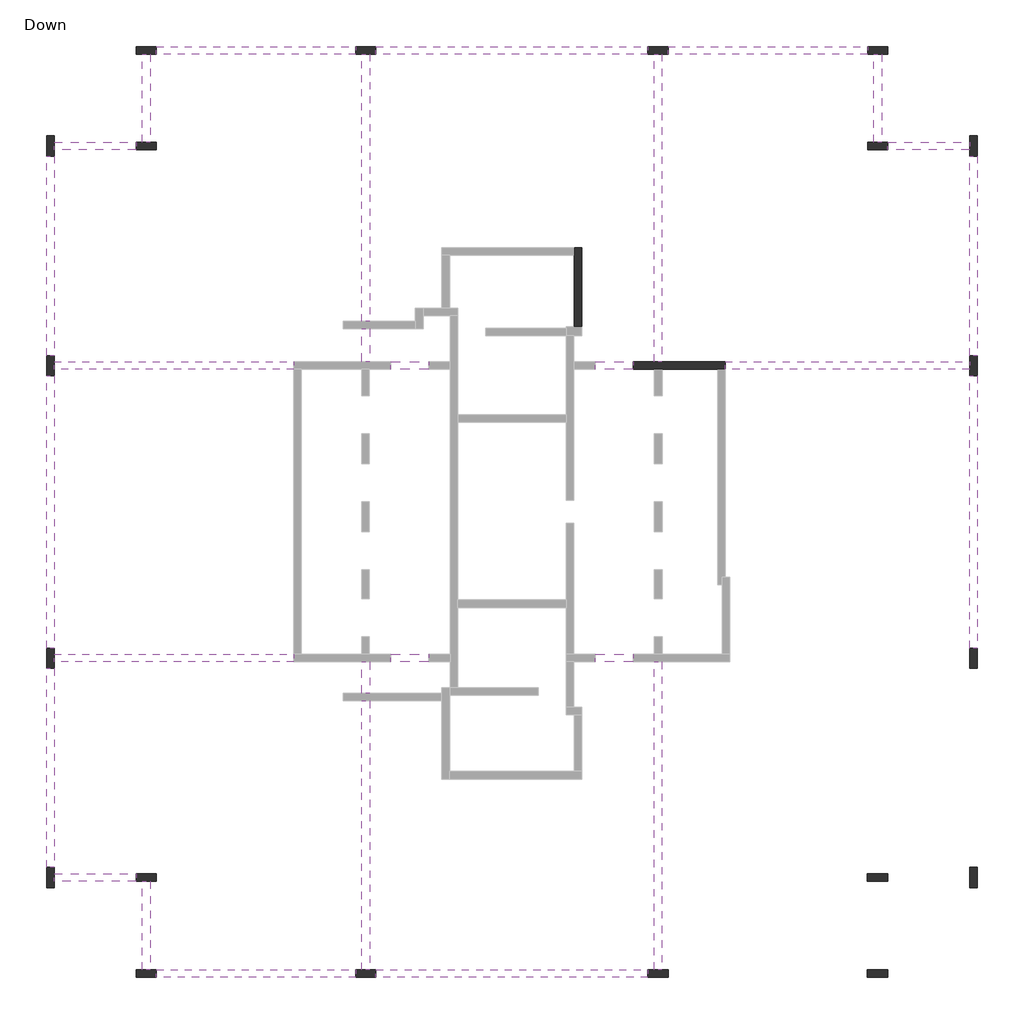
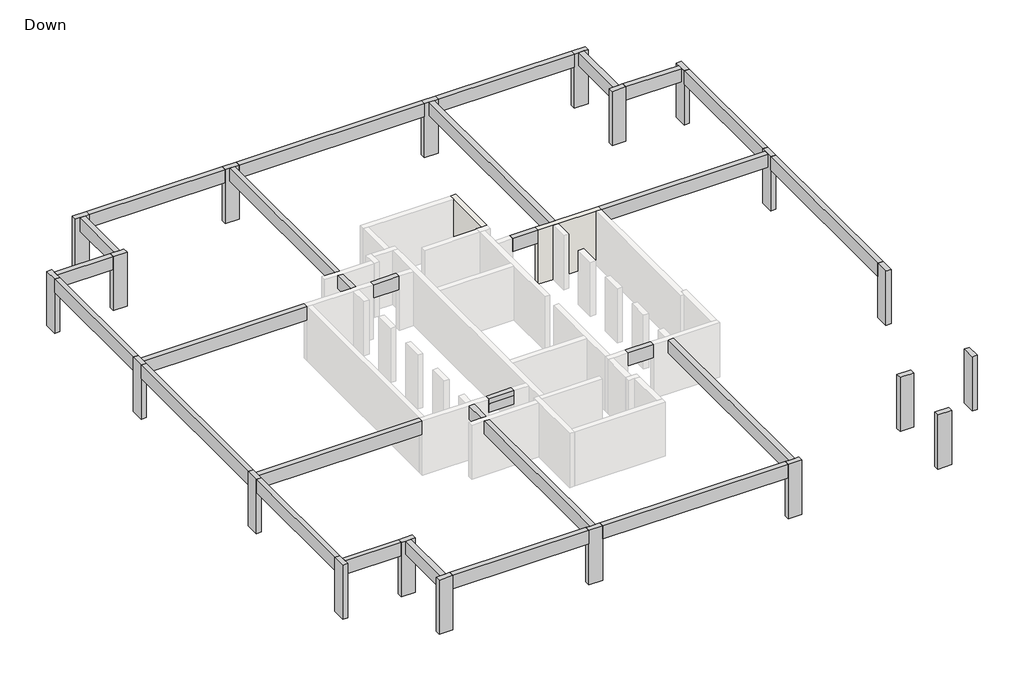
# One storey, part 2 of 2: 29 beams, 20 columns, 2 walls.
"""IFC4 building model written with IfcOpenShell, lengths in millimetres."""

from ifc_helpers import new_model, si_unit, frame, origin, place, context, project, spatial, polyline, outline, extrude, faceted_brep, element, save

model = new_model("IFC4")

# Units and contexts
model_context = context("Model", 3, world=origin())
ifc_project = project(units=[si_unit("LENGTHUNIT", "METRE", prefix="MILLI")], contexts=[model_context])

# Site, building, storey
site = spatial("IfcSite", under=ifc_project)
building = spatial("IfcBuilding", under=site)
storey = spatial("IfcBuildingStorey", under=building, Name="Down", Elevation=0.0)

# Beams
placement = place(None, origin())
element("IfcBeam", 1, ObjectType="Concrete Rectengular Beam : 30/80", at=placement, inside=storey, context=model_context, shape_type="SweptSolid", body=[
    extrude(outline(polyline([(-18816.7874799, -2513.9587131), (-18516.7874799, -2513.9587131), (-18516.7874799, -10341.2814935), (-18816.7874799, -10341.2814935), (-18816.7874799, -2513.9587131)])), frame((0.0, 0.0, 2500.0), z_axis=(0.0, 0.0, 1.0), x_axis=(1.0, 0.0, 0.0)), (0.0, 0.0, 1.0), 800.0),
])
element("IfcBeam", 2, ObjectType="Concrete Rectengular Beam : 30/80", at=placement, inside=storey, context=model_context, shape_type="Brep", body=[
    faceted_brep([(-18516.7874799, -10591.2814935, 3300.0), (-18516.7874799, -10891.2814935, 3300.0), (-15296.5493178, -10891.2814935, 3300.0), (-15296.5493178, -10591.2814935, 3300.0), (-18516.7874799, -10891.2814935, 3000.0), (-18516.7874799, -10891.2814935, 2500.0), (-15296.5493178, -10891.2814935, 2500.0), (-18516.7874799, -10591.2814935, 2500.0), (-15296.5493178, -10591.2814935, 2500.0), (-15296.5493178, -10591.2814935, 3000.0), (-18516.7874799, -10591.2814935, 3000.0)], [[[0, 1, 2, 3]], [[1, 4, 5, 6, 2]], [[5, 7, 8, 6]], [[0, 3, 9, 8, 7, 10]], [[5, 4, 1, 0, 10, 7]], [[3, 2, 6, 8, 9]]]),
])
element("IfcBeam", 3, ObjectType="Concrete Rectengular Beam : 30/80", at=placement, inside=storey, context=model_context, shape_type="Brep", body=[
    faceted_brep([(-14746.5493178, -10891.2814935, 3300.0), (-15046.5493178, -10891.2814935, 3300.0), (-15046.5493178, -14364.3468097, 3300.0), (-14746.5493178, -14364.3468097, 3300.0), (-14746.5493178, -14364.3468097, 3000.0), (-14746.5493178, -14364.3468097, 2500.0), (-14746.5493178, -10891.2814935, 2500.0), (-14746.5493178, -10891.2814935, 3000.0), (-15046.5493178, -10891.2814935, 2500.0), (-15046.5493178, -14364.3468097, 2500.0), (-15046.5493178, -10891.2814935, 3000.0), (-15046.5493178, -14364.3468097, 3000.0)], [[[0, 1, 2, 3]], [[0, 3, 4, 5, 6, 7]], [[8, 6, 5, 9]], [[1, 10, 8, 9, 11, 2]], [[8, 10, 1, 0, 7, 6]], [[3, 2, 11, 9, 5, 4]]]),
])
element("IfcBeam", 4, ObjectType="Concrete Rectengular Beam : 30/80", at=placement, inside=storey, context=model_context, shape_type="SweptSolid", body=[
    extrude(outline(polyline([(-14496.5493178, -14664.3468097), (-14496.5493178, -14364.3468097), (-6665.2243211, -14364.3468097), (-6665.2243211, -14664.3468097), (-14496.5493178, -14664.3468097)])), frame((0.0, 0.0, 2500.0), z_axis=(0.0, 0.0, 1.0), x_axis=(1.0, 0.0, 0.0)), (0.0, 0.0, 1.0), 800.0),
])
element("IfcBeam", 5, ObjectType="Concrete Rectengular Beam : 30/80", at=placement, inside=storey, context=model_context, shape_type="Brep", body=[
    faceted_brep([(-18516.7874799, -1956.2642878, 3300.0), (-18516.7874799, -2256.2642878, 3300.0), (-9097.9299438, -2256.2642878, 3300.0), (-9097.9299438, -1956.2642878, 3300.0), (-18516.7874799, -1956.2642878, 2500.0), (-18516.7874799, -1956.2642878, 3000.0), (-9097.9299438, -1956.2642878, 3000.0), (-9097.9299438, -1956.2642878, 2500.0), (-18516.7874799, -2256.2642878, 2500.0), (-9097.9299438, -2256.2642878, 2500.0), (-18516.7874799, -2256.2642878, 3000.0)], [[[0, 1, 2, 3]], [[4, 5, 0, 3, 6, 7]], [[8, 4, 7, 9]], [[1, 10, 8, 9, 2]], [[8, 10, 1, 0, 5, 4]], [[3, 2, 9, 7, 6]]]),
])
element("IfcBeam", 6, ObjectType="Concrete Rectengular Beam : 30/80", at=placement, inside=storey, context=model_context, shape_type="SweptSolid", body=[
    extrude(outline(polyline([(-18516.7874799, -1713.9587131), (-18816.7874799, -1713.9587131), (-18816.7874799, 8986.0412869), (-18516.7874799, 8986.0412869), (-18516.7874799, -1713.9587131)])), frame((0.0, 0.0, 2500.0), z_axis=(0.0, 0.0, 1.0), x_axis=(1.0, 0.0, 0.0)), (0.0, 0.0, 1.0), 800.0),
])
element("IfcBeam", 7, ObjectType="Concrete Rectengular Beam : 30/80", at=placement, inside=storey, context=model_context, shape_type="Brep", body=[
    faceted_brep([(-18516.7874799, 9551.0309634, 3300.0), (-18516.7874799, 9251.0309634, 3300.0), (-9097.9299438, 9251.0309634, 3300.0), (-9097.9299438, 9551.0309634, 3300.0), (-18516.7874799, 9251.0309634, 3000.0), (-18516.7874799, 9251.0309634, 2500.0), (-9097.9299438, 9251.0309634, 2500.0), (-9097.9299438, 9251.0309634, 3000.0), (-18516.7874799, 9551.0309634, 2500.0), (-9097.9299438, 9551.0309634, 2500.0), (-18516.7874799, 9551.0309634, 3000.0)], [[[0, 1, 2, 3]], [[1, 4, 5, 6, 7, 2]], [[5, 8, 9, 6]], [[8, 10, 0, 3, 9]], [[5, 4, 1, 0, 10, 8]], [[3, 2, 7, 6, 9]]]),
])
element("IfcBeam", 8, ObjectType="Concrete Rectengular Beam : 30/80", at=placement, inside=storey, context=model_context, shape_type="SweptSolid", body=[
    extrude(outline(polyline([(-18516.7874799, 9786.0412869), (-18816.7874799, 9786.0412869), (-18816.7874799, 17624.5114627), (-18516.7874799, 17624.5114627), (-18516.7874799, 9786.0412869)])), frame((0.0, 0.0, 2500.0), z_axis=(0.0, 0.0, 1.0), x_axis=(1.0, 0.0, 0.0)), (0.0, 0.0, 1.0), 800.0),
])
element("IfcBeam", 9, ObjectType="Concrete Rectengular Beam : 30/80", at=placement, inside=storey, context=model_context, shape_type="Brep", body=[
    faceted_brep([(-15046.5493178, 18174.5114627, 3300.0), (-14746.5493178, 18174.5114627, 3300.0), (-14746.5493178, 21634.8017643, 3300.0), (-15046.5493178, 21634.8017643, 3300.0), (-14746.5493178, 18174.5114627, 3000.0), (-14746.5493178, 18174.5114627, 2500.0), (-14746.5493178, 21634.8017643, 2500.0), (-14746.5493178, 21634.8017643, 3000.0), (-15046.5493178, 18174.5114627, 2500.0), (-15046.5493178, 21634.8017643, 2500.0), (-15046.5493178, 18174.5114627, 3000.0), (-15046.5493178, 21634.8017643, 3000.0)], [[[0, 1, 2, 3]], [[2, 1, 4, 5, 6, 7]], [[5, 8, 9, 6]], [[8, 10, 0, 3, 11, 9]], [[1, 0, 10, 8, 5, 4]], [[3, 2, 7, 6, 9, 11]]]),
])
element("IfcBeam", 10, ObjectType="Concrete Rectengular Beam : 30/80", at=placement, inside=storey, context=model_context, shape_type="Brep", body=[
    faceted_brep([(-6115.2243211, 21634.8017643, 3300.0), (-6415.2243211, 21634.8017643, 3300.0), (-6415.2243211, 11137.9545698, 3300.0), (-6115.2243211, 11137.9545698, 3300.0), (-6415.2243211, 21634.8017643, 3000.0), (-6415.2243211, 21634.8017643, 2500.0), (-6415.2243211, 11137.9545698, 2500.0), (-6415.2243211, 11137.9545698, 3000.0), (-6115.2243211, 21634.8017643, 2500.0), (-6115.2243211, 11137.9545698, 2500.0), (-6115.2243211, 21634.8017643, 3000.0), (-6115.2243211, 11137.9545698, 3000.0)], [[[0, 1, 2, 3]], [[1, 4, 5, 6, 7, 2]], [[5, 8, 9, 6]], [[8, 10, 0, 3, 11, 9]], [[1, 0, 10, 8, 5, 4]], [[3, 2, 7, 6, 9, 11]]]),
])
element("IfcBeam", 11, ObjectType="Concrete Rectengular Beam : 30/80", at=placement, inside=storey, context=model_context, shape_type="SweptSolid", body=[
    extrude(outline(polyline([(-5865.2243211, 21634.8017643), (-5865.2243211, 21934.8017643), (4823.25294, 21934.8017643), (4823.25294, 21634.8017643), (-5865.2243211, 21634.8017643)])), frame((0.0, 0.0, 2500.0), z_axis=(0.0, 0.0, 1.0), x_axis=(1.0, 0.0, 0.0)), (0.0, 0.0, 1.0), 800.0),
])
element("IfcBeam", 12, ObjectType="Concrete Rectengular Beam : 30/80", at=placement, inside=storey, context=model_context, shape_type="Brep", body=[
    faceted_brep([(14014.5779368, 21634.8017643, 3300.0), (13714.5779368, 21634.8017643, 3300.0), (13714.5779368, 18174.5114627, 3300.0), (14014.5779368, 18174.5114627, 3300.0), (13714.5779368, 21634.8017643, 3000.0), (13714.5779368, 21634.8017643, 2500.0), (13714.5779368, 18174.5114627, 2500.0), (13714.5779368, 18174.5114627, 3000.0), (14014.5779368, 21634.8017643, 2500.0), (14014.5779368, 18174.5114627, 2500.0), (14014.5779368, 21634.8017643, 3000.0), (14014.5779368, 18174.5114627, 3000.0)], [[[0, 1, 2, 3]], [[2, 1, 4, 5, 6, 7]], [[5, 8, 9, 6]], [[8, 10, 0, 3, 11, 9]], [[1, 0, 10, 8, 5, 4]], [[3, 2, 7, 6, 9, 11]]]),
])
element("IfcBeam", 13, ObjectType="Concrete Rectengular Beam : 30/80", at=placement, inside=storey, context=model_context, shape_type="SweptSolid", body=[
    extrude(outline(polyline([(17474.8160989, 17624.5114627), (17774.8160989, 17624.5114627), (17774.8160989, 9786.0412869), (17474.8160989, 9786.0412869), (17474.8160989, 17624.5114627)])), frame((0.0, 0.0, 2500.0), z_axis=(0.0, 0.0, 1.0), x_axis=(1.0, 0.0, 0.0)), (0.0, 0.0, 1.0), 800.0),
])
element("IfcBeam", 14, ObjectType="Concrete Rectengular Beam : 30/80", at=placement, inside=storey, context=model_context, shape_type="SweptSolid", body=[
    extrude(outline(polyline([(17774.8160989, -1713.9587131), (17474.8160989, -1713.9587131), (17474.8160989, 8986.0412869), (17774.8160989, 8986.0412869), (17774.8160989, -1713.9587131)])), frame((0.0, 0.0, 2500.0), z_axis=(0.0, 0.0, 1.0), x_axis=(1.0, 0.0, 0.0)), (0.0, 0.0, 1.0), 800.0),
])
element("IfcBeam", 15, ObjectType="Concrete Rectengular Beam : 30/80", at=placement, inside=storey, context=model_context, shape_type="Brep", body=[
    faceted_brep([(14264.5779368, 18174.5114627, 3300.0), (14264.5779368, 17874.5114627, 3300.0), (17474.8160989, 17874.5114627, 3300.0), (17474.8160989, 18174.5114627, 3300.0), (14264.5779368, 18174.5114627, 2500.0), (17474.8160989, 18174.5114627, 3000.0), (17474.8160989, 18174.5114627, 2500.0), (14264.5779368, 17874.5114627, 2500.0), (17474.8160989, 17874.5114627, 2500.0), (14264.5779368, 17874.5114627, 3000.0), (17474.8160989, 17874.5114627, 3000.0)], [[[0, 1, 2, 3]], [[4, 0, 3, 5, 6]], [[7, 4, 6, 8]], [[2, 1, 9, 7, 8, 10]], [[1, 0, 4, 7, 9]], [[6, 5, 3, 2, 10, 8]]]),
])
element("IfcBeam", 16, ObjectType="Concrete Rectengular Beam : 30/80", at=placement, inside=storey, context=model_context, shape_type="SweptSolid", body=[
    extrude(outline(polyline([(5623.25294, 21634.8017643), (5623.25294, 21934.8017643), (13464.5779368, 21934.8017643), (13464.5779368, 21634.8017643), (5623.25294, 21634.8017643)])), frame((0.0, 0.0, 2500.0), z_axis=(0.0, 0.0, 1.0), x_axis=(1.0, 0.0, 0.0)), (0.0, 0.0, 1.0), 800.0),
])
element("IfcBeam", 17, ObjectType="Concrete Rectengular Beam : 30/80", at=placement, inside=storey, context=model_context, shape_type="SweptSolid", body=[
    extrude(outline(polyline([(-5865.2243211, -14664.3468097), (-5865.2243211, -14364.3468097), (4823.25294, -14364.3468097), (4823.25294, -14664.3468097), (-5865.2243211, -14664.3468097)])), frame((0.0, 0.0, 2500.0), z_axis=(0.0, 0.0, 1.0), x_axis=(1.0, 0.0, 0.0)), (0.0, 0.0, 1.0), 800.0),
])
element("IfcBeam", 18, ObjectType="Concrete Rectengular Beam : 30/80", at=placement, inside=storey, context=model_context, shape_type="Brep", body=[
    faceted_brep([(-6415.2243211, -14364.3468097, 3300.0), (-6115.2243211, -14364.3468097, 3300.0), (-6115.2243211, -3792.8093669, 3300.0), (-6415.2243211, -3792.8093669, 3300.0), (-6115.2243211, -14364.3468097, 3000.0), (-6115.2243211, -14364.3468097, 2500.0), (-6115.2243211, -3792.8093669, 2500.0), (-6115.2243211, -3792.8093669, 3000.0), (-6415.2243211, -14364.3468097, 2500.0), (-6415.2243211, -3792.8093669, 2500.0), (-6415.2243211, -14364.3468097, 3000.0), (-6415.2243211, -3792.8093669, 3000.0)], [[[0, 1, 2, 3]], [[1, 4, 5, 6, 7, 2]], [[5, 8, 9, 6]], [[8, 10, 0, 3, 11, 9]], [[0, 10, 8, 5, 4, 1]], [[3, 2, 7, 6, 9, 11]]]),
])
element("IfcBeam", 19, ObjectType="Concrete Rectengular Beam : 30/80", at=placement, inside=storey, context=model_context, shape_type="Brep", body=[
    faceted_brep([(-6115.2243211, -2256.2642878, 3300.0), (-6415.2243211, -2256.2642878, 3300.0), (-6415.2243211, -3492.8093669, 3300.0), (-6115.2243211, -3492.8093669, 3300.0), (-6115.2243211, -2256.2642878, 2500.0), (-6115.2243211, -2256.2642878, 3000.0), (-6115.2243211, -3492.8093669, 3000.0), (-6115.2243211, -3492.8093669, 2500.0), (-6415.2243211, -2256.2642878, 2500.0), (-6415.2243211, -3492.8093669, 2500.0), (-6415.2243211, -2256.2642878, 3000.0), (-6415.2243211, -3492.8093669, 3000.0)], [[[0, 1, 2, 3]], [[4, 5, 0, 3, 6, 7]], [[8, 4, 7, 9]], [[1, 10, 8, 9, 11, 2]], [[1, 0, 5, 4, 8, 10]], [[3, 2, 11, 9, 7, 6]]]),
])
element("IfcBeam", 20, ObjectType="Concrete Rectengular Beam : 30/80", at=placement, inside=storey, context=model_context, shape_type="Brep", body=[
    faceted_brep([(5073.25294, -14364.3468097, 3300.0), (5373.25294, -14364.3468097, 3300.0), (5373.25294, -2256.2642878, 3300.0), (5073.25294, -2256.2642878, 3300.0), (5073.25294, -14364.3468097, 2500.0), (5073.25294, -14364.3468097, 3000.0), (5073.25294, -2256.2642878, 3000.0), (5073.25294, -2256.2642878, 2500.0), (5373.25294, -14364.3468097, 2500.0), (5373.25294, -2256.2642878, 2500.0), (5373.25294, -14364.3468097, 3000.0), (5373.25294, -2256.2642878, 3000.0)], [[[0, 1, 2, 3]], [[4, 5, 0, 3, 6, 7]], [[8, 4, 7, 9]], [[1, 10, 8, 9, 11, 2]], [[8, 10, 1, 0, 5, 4]], [[3, 2, 11, 9, 7, 6]]]),
])
element("IfcBeam", 21, ObjectType="Concrete Rectengular Beam : 30/80", at=placement, inside=storey, context=model_context, shape_type="Brep", body=[
    faceted_brep([(-18516.7874799, 18174.5114627, 3300.0), (-18516.7874799, 17874.5114627, 3300.0), (-15296.5493178, 17874.5114627, 3300.0), (-15296.5493178, 18174.5114627, 3300.0), (-18516.7874799, 17874.5114627, 3000.0), (-18516.7874799, 17874.5114627, 2500.0), (-15296.5493178, 17874.5114627, 2500.0), (-15296.5493178, 17874.5114627, 3000.0), (-18516.7874799, 18174.5114627, 2500.0), (-15296.5493178, 18174.5114627, 2500.0), (-18516.7874799, 18174.5114627, 3000.0)], [[[0, 1, 2, 3]], [[2, 1, 4, 5, 6, 7]], [[5, 8, 9, 6]], [[8, 10, 0, 3, 9]], [[0, 10, 8, 5, 4, 1]], [[3, 2, 7, 6, 9]]]),
])
element("IfcBeam", 22, ObjectType="Concrete Rectengular Beam : 30/80", at=placement, inside=storey, context=model_context, shape_type="SweptSolid", body=[
    extrude(outline(polyline([(-14496.5493178, 21634.8017643), (-14496.5493178, 21934.8017643), (-6665.2243211, 21934.8017643), (-6665.2243211, 21634.8017643), (-14496.5493178, 21634.8017643)])), frame((0.0, 0.0, 2500.0), z_axis=(0.0, 0.0, 1.0), x_axis=(1.0, 0.0, 0.0)), (0.0, 0.0, 1.0), 800.0),
])
element("IfcBeam", 23, ObjectType="Concrete Rectengular Beam : 30/80", at=placement, inside=storey, context=model_context, shape_type="Brep", body=[
    faceted_brep([(5373.25294, 21634.8017643, 3300.0), (5073.25294, 21634.8017643, 3300.0), (5073.25294, 9551.0309634, 3300.0), (5373.25294, 9551.0309634, 3300.0), (5073.25294, 21634.8017643, 3000.0), (5073.25294, 21634.8017643, 2500.0), (5073.25294, 9551.0309634, 2500.0), (5073.25294, 9551.0309634, 3000.0), (5373.25294, 21634.8017643, 2500.0), (5373.25294, 9551.0309634, 2500.0), (5373.25294, 21634.8017643, 3000.0), (5373.25294, 9551.0309634, 3000.0)], [[[0, 1, 2, 3]], [[1, 4, 5, 6, 7, 2]], [[5, 8, 9, 6]], [[8, 10, 0, 3, 11, 9]], [[5, 4, 1, 0, 10, 8]], [[3, 2, 7, 6, 9, 11]]]),
])
element("IfcBeam", 24, ObjectType="Concrete Rectengular Beam : 30/80", at=placement, inside=storey, context=model_context, shape_type="Brep", body=[
    faceted_brep([(17474.8160989, 9251.0309634, 3300.0), (17474.8160989, 9551.0309634, 3300.0), (7862.8408752, 9551.0309634, 3300.0), (7862.8408752, 9251.0309634, 3300.0), (17474.8160989, 9551.0309634, 3000.0), (17474.8160989, 9551.0309634, 2500.0), (7862.8408752, 9551.0309634, 2500.0), (17474.8160989, 9251.0309634, 2500.0), (7862.8408752, 9251.0309634, 2500.0), (17474.8160989, 9251.0309634, 3000.0), (7862.8408752, 9251.0309634, 3000.0)], [[[0, 1, 2, 3]], [[1, 4, 5, 6, 2]], [[5, 7, 8, 6]], [[7, 9, 0, 3, 10, 8]], [[5, 4, 1, 0, 9, 7]], [[3, 2, 6, 8, 10]]]),
])
element("IfcBeam", 25, ObjectType="Concrete Rectengular Beam : 30/80", at=placement, inside=storey, context=model_context, shape_type="SweptSolid", body=[
    extrude(outline(polyline([(2756.2889137, 9251.0309634), (2756.2889137, 9551.0309634), (4242.4554657, 9551.0309634), (4242.4554657, 9251.0309634), (2756.2889137, 9251.0309634)])), frame((0.0, 0.0, 2500.0), z_axis=(0.0, 0.0, 1.0), x_axis=(1.0, 0.0, 0.0)), (0.0, 0.0, 1.0), 800.0),
])
element("IfcBeam", 26, ObjectType="Concrete Rectengular Beam : 30/80", at=placement, inside=storey, context=model_context, shape_type="SweptSolid", body=[
    extrude(outline(polyline([(2756.2889137, -2256.2642878), (2756.2889137, -1956.2642878), (4242.4554657, -1956.2642878), (4242.4554657, -2256.2642878), (2756.2889137, -2256.2642878)])), frame((0.0, 0.0, 2500.0), z_axis=(0.0, 0.0, 1.0), x_axis=(1.0, 0.0, 0.0)), (0.0, 0.0, 1.0), 800.0),
])
element("IfcBeam", 27, ObjectType="Concrete Rectengular Beam : 30/80", at=placement, inside=storey, context=model_context, shape_type="SweptSolid", body=[
    extrude(outline(polyline([(-1956.2642878, 3300.0), (-1956.2642878, 2500.0), (-2256.2642878, 2500.0), (-2256.2642878, 3000.0), (-2251.2642878, 3000.0), (-2251.2642878, 3300.0), (-1956.2642878, 3300.0)])), frame((-5277.5582989, 0.0, 0.0), z_axis=(1.0, 0.0, 0.0), x_axis=(0.0, 1.0, 0.0)), (0.0, 0.0, 1.0), 1486.166552),
])
element("IfcBeam", 28, ObjectType="Concrete Rectengular Beam : 30/80", at=placement, inside=storey, context=model_context, shape_type="SweptSolid", body=[
    extrude(outline(polyline([(-3791.391747, 9551.0309634), (-3791.391747, 9251.0309634), (-5277.5582989, 9251.0309634), (-5277.5582989, 9551.0309634), (-3791.391747, 9551.0309634)])), frame((0.0, 0.0, 2500.0), z_axis=(0.0, 0.0, 1.0), x_axis=(1.0, 0.0, 0.0)), (0.0, 0.0, 1.0), 800.0),
])
element("IfcBeam", 29, ObjectType="Concrete Rectengular Beam : 30/80", at=placement, inside=storey, context=model_context, shape_type="Brep", body=[
    faceted_brep([(-6415.2243211, 9551.0309634, 3300.0), (-6115.2243211, 9551.0309634, 3300.0), (-6115.2243211, 10837.9545698, 3300.0), (-6415.2243211, 10837.9545698, 3300.0), (-6115.2243211, 9551.0309634, 3000.0), (-6115.2243211, 9551.0309634, 2500.0), (-6115.2243211, 10837.9545698, 2500.0), (-6115.2243211, 10837.9545698, 3000.0), (-6415.2243211, 9551.0309634, 2500.0), (-6415.2243211, 10837.9545698, 2500.0), (-6415.2243211, 9551.0309634, 3000.0), (-6415.2243211, 10837.9545698, 3000.0)], [[[0, 1, 2, 3]], [[1, 4, 5, 6, 7, 2]], [[5, 8, 9, 6]], [[8, 10, 0, 3, 11, 9]], [[1, 0, 10, 8, 5, 4]], [[3, 2, 7, 6, 9, 11]]]),
])

# Columns
element("IfcColumn", 30, ObjectType="Concrete Rectengular Column : 30/80", at=placement, inside=storey, context=model_context, shape_type="Brep", body=[
    faceted_brep([(-18516.7874799, -1713.9587131, 0.0), (-18516.7874799, -2513.9587131, 0.0), (-18816.7874799, -2513.9587131, 0.0), (-18816.7874799, -1713.9587131, 0.0), (-18516.7874799, -1713.9587131, 3300.0), (-18516.7874799, -1956.2642878, 3300.0), (-18516.7874799, -2256.2642878, 3300.0), (-18516.7874799, -2513.9587131, 3300.0), (-18816.7874799, -2513.9587131, 3300.0), (-18816.7874799, -1713.9587131, 3300.0)], [[[0, 1, 2, 3]], [[4, 5, 6, 7, 1, 0]], [[7, 8, 2, 1]], [[8, 9, 3, 2]], [[9, 4, 0, 3]], [[4, 9, 8, 7, 6, 5]]]),
])
element("IfcColumn", 31, ObjectType="Concrete Rectengular Column : 30/80", at=placement, inside=storey, context=model_context, shape_type="Brep", body=[
    faceted_brep([(-18516.7874799, -10341.2814935, 0.0), (-18516.7874799, -11141.2814935, 0.0), (-18816.7874799, -11141.2814935, 0.0), (-18816.7874799, -10341.2814935, 0.0), (-18516.7874799, -10341.2814935, 3300.0), (-18516.7874799, -10591.2814935, 3300.0), (-18516.7874799, -10891.2814935, 3300.0), (-18516.7874799, -11141.2814935, 3300.0), (-18516.7874799, -11141.2814935, 3000.0), (-18816.7874799, -11141.2814935, 3300.0), (-18816.7874799, -11141.2814935, 3000.0), (-18816.7874799, -10341.2814935, 3300.0)], [[[0, 1, 2, 3]], [[4, 5, 6, 7, 8, 1, 0]], [[7, 9, 10, 2, 1, 8]], [[9, 11, 3, 2, 10]], [[11, 4, 0, 3]], [[4, 11, 9, 7, 6, 5]]]),
])
element("IfcColumn", 32, ObjectType="Concrete Rectengular Column : 30/80", at=placement, inside=storey, context=model_context, shape_type="Brep", body=[
    faceted_brep([(-15296.5493178, -10591.2814935, 0.0), (-14496.5493178, -10591.2814935, 0.0), (-14496.5493178, -10891.2814935, 0.0), (-15296.5493178, -10891.2814935, 0.0), (-15296.5493178, -10591.2814935, 3300.0), (-14496.5493178, -10591.2814935, 3300.0), (-14496.5493178, -10591.2814935, 3000.0), (-14496.5493178, -10891.2814935, 3300.0), (-14496.5493178, -10891.2814935, 3000.0), (-14746.5493178, -10891.2814935, 3300.0), (-15046.5493178, -10891.2814935, 3300.0), (-15296.5493178, -10891.2814935, 3300.0)], [[[0, 1, 2, 3]], [[4, 5, 6, 1, 0]], [[5, 7, 8, 2, 1, 6]], [[7, 9, 10, 11, 3, 2, 8]], [[11, 4, 0, 3]], [[4, 11, 10, 9, 7, 5]]]),
])
element("IfcColumn", 33, ObjectType="Concrete Rectengular Column : 30/80", at=placement, inside=storey, context=model_context, shape_type="Brep", body=[
    faceted_brep([(-15296.5493178, -14364.3468097, 0.0), (-14496.5493178, -14364.3468097, 0.0), (-14496.5493178, -14664.3468097, 0.0), (-15296.5493178, -14664.3468097, 0.0), (-15296.5493178, -14364.3468097, 3300.0), (-15046.5493178, -14364.3468097, 3300.0), (-14746.5493178, -14364.3468097, 3300.0), (-14496.5493178, -14364.3468097, 3300.0), (-15296.5493178, -14364.3468097, 3000.0), (-14496.5493178, -14664.3468097, 3300.0), (-15296.5493178, -14664.3468097, 3300.0), (-15296.5493178, -14664.3468097, 3000.0)], [[[0, 1, 2, 3]], [[4, 5, 6, 7, 1, 0, 8]], [[7, 9, 2, 1]], [[9, 10, 11, 3, 2]], [[10, 4, 8, 0, 3, 11]], [[4, 10, 9, 7, 6, 5]]]),
])
element("IfcColumn", 34, ObjectType="Concrete Rectengular Column : 30/80", at=placement, inside=storey, context=model_context, shape_type="Brep", body=[
    faceted_brep([(-6665.2243211, -14364.3468097, 0.0), (-5865.2243211, -14364.3468097, 0.0), (-5865.2243211, -14664.3468097, 0.0), (-6665.2243211, -14664.3468097, 0.0), (-6665.2243211, -14364.3468097, 3300.0), (-6415.2243211, -14364.3468097, 3300.0), (-6115.2243211, -14364.3468097, 3300.0), (-5865.2243211, -14364.3468097, 3300.0), (-5865.2243211, -14664.3468097, 3300.0), (-6665.2243211, -14664.3468097, 3300.0)], [[[0, 1, 2, 3]], [[4, 5, 6, 7, 1, 0]], [[7, 8, 2, 1]], [[8, 9, 3, 2]], [[9, 4, 0, 3]], [[4, 9, 8, 7, 6, 5]]]),
])
element("IfcColumn", 35, ObjectType="Concrete Rectengular Column : 30/80", at=placement, inside=storey, context=model_context, shape_type="Brep", body=[
    faceted_brep([(17474.8160989, -1713.9587131, 0.0), (17774.8160989, -1713.9587131, 0.0), (17774.8160989, -2513.9587131, 0.0), (17474.8160989, -2513.9587131, 0.0), (17474.8160989, -1713.9587131, 3300.0), (17474.8160989, -2513.9587131, 3300.0), (17474.8160989, -2256.2642878, 3300.0), (17474.8160989, -1956.2642878, 3300.0), (17774.8160989, -2513.9587131, 3300.0), (17774.8160989, -1713.9587131, 3300.0)], [[[0, 1, 2, 3]], [[4, 0, 3, 5, 6, 7]], [[5, 3, 2, 8]], [[8, 2, 1, 9]], [[9, 1, 0, 4]], [[4, 7, 6, 5, 8, 9]]]),
])
element("IfcColumn", 36, ObjectType="Concrete Rectengular Column : 30/80", at=placement, inside=storey, context=model_context, shape_type="Brep", body=[
    faceted_brep([(17474.8160989, -10341.2814935, 0.0), (17774.8160989, -10341.2814935, 0.0), (17774.8160989, -11141.2814935, 0.0), (17474.8160989, -11141.2814935, 0.0), (17474.8160989, -10341.2814935, 3300.0), (17474.8160989, -11141.2814935, 3000.0), (17474.8160989, -11141.2814935, 3300.0), (17474.8160989, -10891.2814935, 3300.0), (17474.8160989, -10591.2814935, 3300.0), (17774.8160989, -11141.2814935, 3000.0), (17774.8160989, -11141.2814935, 3300.0), (17774.8160989, -10341.2814935, 3300.0)], [[[0, 1, 2, 3]], [[4, 0, 3, 5, 6, 7, 8]], [[6, 5, 3, 2, 9, 10]], [[10, 9, 2, 1, 11]], [[11, 1, 0, 4]], [[4, 8, 7, 6, 10, 11]]]),
])
element("IfcColumn", 37, ObjectType="Concrete Rectengular Column : 30/80", at=placement, inside=storey, context=model_context, shape_type="Brep", body=[
    faceted_brep([(14254.5779368, -10591.2814935, 0.0), (14254.5779368, -10891.2814935, 0.0), (13454.5779368, -10891.2814935, 0.0), (13454.5779368, -10591.2814935, 0.0), (14254.5779368, -10591.2814935, 3300.0), (13454.5779368, -10591.2814935, 3000.0), (13454.5779368, -10591.2814935, 3300.0), (13454.5779368, -10891.2814935, 3000.0), (13454.5779368, -10891.2814935, 3300.0), (14254.5779368, -10891.2814935, 3300.0), (14004.5779368, -10891.2814935, 3300.0), (13704.5779368, -10891.2814935, 3300.0)], [[[0, 1, 2, 3]], [[4, 0, 3, 5, 6]], [[6, 5, 3, 2, 7, 8]], [[8, 7, 2, 1, 9, 10, 11]], [[9, 1, 0, 4]], [[4, 6, 8, 11, 10, 9]]]),
])
element("IfcColumn", 38, ObjectType="Concrete Rectengular Column : 30/80", at=placement, inside=storey, context=model_context, shape_type="Brep", body=[
    faceted_brep([(14254.5779368, -14364.3468097, 0.0), (14254.5779368, -14664.3468097, 0.0), (13454.5779368, -14664.3468097, 0.0), (13454.5779368, -14364.3468097, 0.0), (14254.5779368, -14364.3468097, 3300.0), (14254.5779368, -14364.3468097, 3000.0), (13454.5779368, -14364.3468097, 3300.0), (13704.5779368, -14364.3468097, 3300.0), (14004.5779368, -14364.3468097, 3300.0), (13454.5779368, -14664.3468097, 3300.0), (14254.5779368, -14664.3468097, 3000.0), (14254.5779368, -14664.3468097, 3300.0)], [[[0, 1, 2, 3]], [[4, 5, 0, 3, 6, 7, 8]], [[6, 3, 2, 9]], [[9, 2, 1, 10, 11]], [[11, 10, 1, 0, 5, 4]], [[4, 8, 7, 6, 9, 11]]]),
])
element("IfcColumn", 39, ObjectType="Concrete Rectengular Column : 30/80", at=placement, inside=storey, context=model_context, shape_type="Brep", body=[
    faceted_brep([(5623.25294, -14364.3468097, 0.0), (5623.25294, -14664.3468097, 0.0), (4823.25294, -14664.3468097, 0.0), (4823.25294, -14364.3468097, 0.0), (5623.25294, -14364.3468097, 3300.0), (4823.25294, -14364.3468097, 3300.0), (5073.25294, -14364.3468097, 3300.0), (5373.25294, -14364.3468097, 3300.0), (4823.25294, -14664.3468097, 3300.0), (5623.25294, -14664.3468097, 3300.0)], [[[0, 1, 2, 3]], [[4, 0, 3, 5, 6, 7]], [[5, 3, 2, 8]], [[8, 2, 1, 9]], [[9, 1, 0, 4]], [[4, 7, 6, 5, 8, 9]]]),
])
element("IfcColumn", 40, ObjectType="Concrete Rectengular Column : 30/80", at=placement, inside=storey, context=model_context, shape_type="Brep", body=[
    faceted_brep([(-18516.7874799, 9786.0412869, 0.0), (-18516.7874799, 8986.0412869, 0.0), (-18816.7874799, 8986.0412869, 0.0), (-18816.7874799, 9786.0412869, 0.0), (-18516.7874799, 9786.0412869, 3300.0), (-18516.7874799, 9551.0309634, 3300.0), (-18516.7874799, 9251.0309634, 3300.0), (-18516.7874799, 8986.0412869, 3300.0), (-18516.7874799, 8986.0412869, 2500.0), (-18816.7874799, 8986.0412869, 3300.0), (-18816.7874799, 8986.0412869, 2500.0), (-18816.7874799, 9786.0412869, 3300.0)], [[[0, 1, 2, 3]], [[4, 5, 6, 7, 8, 1, 0]], [[7, 9, 10, 2, 1, 8]], [[9, 11, 3, 2, 10]], [[11, 4, 0, 3]], [[4, 11, 9, 7, 6, 5]]]),
])
element("IfcColumn", 41, ObjectType="Concrete Rectengular Column : 30/80", at=placement, inside=storey, context=model_context, shape_type="Brep", body=[
    faceted_brep([(-18516.7874799, 18424.5114627, 0.0), (-18516.7874799, 17624.5114627, 0.0), (-18816.7874799, 17624.5114627, 0.0), (-18816.7874799, 18424.5114627, 0.0), (-18516.7874799, 18424.5114627, 3300.0), (-18516.7874799, 18174.5114627, 3300.0), (-18516.7874799, 17874.5114627, 3300.0), (-18516.7874799, 17624.5114627, 3300.0), (-18516.7874799, 18424.5114627, 3000.0), (-18816.7874799, 17624.5114627, 3300.0), (-18816.7874799, 18424.5114627, 3300.0), (-18816.7874799, 18424.5114627, 3000.0)], [[[0, 1, 2, 3]], [[4, 5, 6, 7, 1, 0, 8]], [[7, 9, 2, 1]], [[9, 10, 11, 3, 2]], [[10, 4, 8, 0, 3, 11]], [[4, 10, 9, 7, 6, 5]]]),
])
element("IfcColumn", 42, ObjectType="Concrete Rectengular Column : 30/80", at=placement, inside=storey, context=model_context, shape_type="Brep", body=[
    faceted_brep([(-15296.5493178, 18174.5114627, 0.0), (-14496.5493178, 18174.5114627, 0.0), (-14496.5493178, 17874.5114627, 0.0), (-15296.5493178, 17874.5114627, 0.0), (-15296.5493178, 18174.5114627, 3300.0), (-15046.5493178, 18174.5114627, 3300.0), (-14746.5493178, 18174.5114627, 3300.0), (-14496.5493178, 18174.5114627, 3300.0), (-14496.5493178, 18174.5114627, 3000.0), (-14496.5493178, 17874.5114627, 3300.0), (-14496.5493178, 17874.5114627, 3000.0), (-15296.5493178, 17874.5114627, 3300.0)], [[[0, 1, 2, 3]], [[4, 5, 6, 7, 8, 1, 0]], [[7, 9, 10, 2, 1, 8]], [[9, 11, 3, 2, 10]], [[11, 4, 0, 3]], [[4, 11, 9, 7, 6, 5]]]),
])
element("IfcColumn", 43, ObjectType="Concrete Rectengular Column : 30/80", at=placement, inside=storey, context=model_context, shape_type="Brep", body=[
    faceted_brep([(-15296.5493178, 21934.8017643, 0.0), (-14496.5493178, 21934.8017643, 0.0), (-14496.5493178, 21634.8017643, 0.0), (-15296.5493178, 21634.8017643, 0.0), (-15296.5493178, 21934.8017643, 3300.0), (-14496.5493178, 21934.8017643, 3300.0), (-15296.5493178, 21934.8017643, 3000.0), (-14496.5493178, 21634.8017643, 3300.0), (-14746.5493178, 21634.8017643, 3300.0), (-15046.5493178, 21634.8017643, 3300.0), (-15296.5493178, 21634.8017643, 3300.0), (-15296.5493178, 21634.8017643, 3000.0)], [[[0, 1, 2, 3]], [[4, 5, 1, 0, 6]], [[5, 7, 2, 1]], [[7, 8, 9, 10, 11, 3, 2]], [[10, 4, 6, 0, 3, 11]], [[4, 10, 9, 8, 7, 5]]]),
])
element("IfcColumn", 44, ObjectType="Concrete Rectengular Column : 30/80", at=placement, inside=storey, context=model_context, shape_type="Brep", body=[
    faceted_brep([(-6665.2243211, 21934.8017643, 0.0), (-5865.2243211, 21934.8017643, 0.0), (-5865.2243211, 21634.8017643, 0.0), (-6665.2243211, 21634.8017643, 0.0), (-6665.2243211, 21934.8017643, 3300.0), (-5865.2243211, 21934.8017643, 3300.0), (-5865.2243211, 21634.8017643, 3300.0), (-6115.2243211, 21634.8017643, 3300.0), (-6415.2243211, 21634.8017643, 3300.0), (-6665.2243211, 21634.8017643, 3300.0)], [[[0, 1, 2, 3]], [[4, 5, 1, 0]], [[5, 6, 2, 1]], [[6, 7, 8, 9, 3, 2]], [[9, 4, 0, 3]], [[4, 9, 8, 7, 6, 5]]]),
])
element("IfcColumn", 45, ObjectType="Concrete Rectengular Column : 30/80", at=placement, inside=storey, context=model_context, shape_type="Brep", body=[
    faceted_brep([(4823.25294, 21934.8017643, 0.0), (5623.25294, 21934.8017643, 0.0), (5623.25294, 21634.8017643, 0.0), (4823.25294, 21634.8017643, 0.0), (4823.25294, 21934.8017643, 3300.0), (5623.25294, 21934.8017643, 3300.0), (5623.25294, 21634.8017643, 3300.0), (5373.25294, 21634.8017643, 3300.0), (5073.25294, 21634.8017643, 3300.0), (4823.25294, 21634.8017643, 3300.0)], [[[0, 1, 2, 3]], [[4, 5, 1, 0]], [[5, 6, 2, 1]], [[6, 7, 8, 9, 3, 2]], [[9, 4, 0, 3]], [[4, 9, 8, 7, 6, 5]]]),
])
element("IfcColumn", 46, ObjectType="Concrete Rectengular Column : 30/80", at=placement, inside=storey, context=model_context, shape_type="Brep", body=[
    faceted_brep([(13464.5779368, 21934.8017643, 0.0), (14264.5779368, 21934.8017643, 0.0), (14264.5779368, 21634.8017643, 0.0), (13464.5779368, 21634.8017643, 0.0), (13464.5779368, 21934.8017643, 3300.0), (14264.5779368, 21934.8017643, 3300.0), (14264.5779368, 21934.8017643, 3000.0), (14264.5779368, 21634.8017643, 3300.0), (14264.5779368, 21634.8017643, 3000.0), (14014.5779368, 21634.8017643, 3300.0), (13714.5779368, 21634.8017643, 3300.0), (13464.5779368, 21634.8017643, 3300.0)], [[[0, 1, 2, 3]], [[4, 5, 6, 1, 0]], [[5, 7, 8, 2, 1, 6]], [[7, 9, 10, 11, 3, 2, 8]], [[11, 4, 0, 3]], [[4, 11, 10, 9, 7, 5]]]),
])
element("IfcColumn", 47, ObjectType="Concrete Rectengular Column : 30/80", at=placement, inside=storey, context=model_context, shape_type="Brep", body=[
    faceted_brep([(13464.5779368, 18174.5114627, 0.0), (14264.5779368, 18174.5114627, 0.0), (14264.5779368, 17874.5114627, 0.0), (13464.5779368, 17874.5114627, 0.0), (13464.5779368, 18174.5114627, 3300.0), (13714.5779368, 18174.5114627, 3300.0), (14014.5779368, 18174.5114627, 3300.0), (14264.5779368, 18174.5114627, 3300.0), (13464.5779368, 18174.5114627, 3000.0), (14264.5779368, 17874.5114627, 3300.0), (13464.5779368, 17874.5114627, 3300.0), (13464.5779368, 17874.5114627, 3000.0)], [[[0, 1, 2, 3]], [[4, 5, 6, 7, 1, 0, 8]], [[7, 9, 2, 1]], [[9, 10, 11, 3, 2]], [[10, 4, 8, 0, 3, 11]], [[4, 10, 9, 7, 6, 5]]]),
])
element("IfcColumn", 48, ObjectType="Concrete Rectengular Column : 30/80", at=placement, inside=storey, context=model_context, shape_type="Brep", body=[
    faceted_brep([(17474.8160989, 17624.5114627, 0.0), (17474.8160989, 18424.5114627, 0.0), (17774.8160989, 18424.5114627, 0.0), (17774.8160989, 17624.5114627, 0.0), (17474.8160989, 17624.5114627, 3300.0), (17474.8160989, 17874.5114627, 3300.0), (17474.8160989, 18174.5114627, 3300.0), (17474.8160989, 18424.5114627, 3300.0), (17474.8160989, 18424.5114627, 3000.0), (17774.8160989, 18424.5114627, 3300.0), (17774.8160989, 18424.5114627, 3000.0), (17774.8160989, 17624.5114627, 3300.0)], [[[0, 1, 2, 3]], [[4, 5, 6, 7, 8, 1, 0]], [[7, 9, 10, 2, 1, 8]], [[9, 11, 3, 2, 10]], [[11, 4, 0, 3]], [[4, 11, 9, 7, 6, 5]]]),
])
element("IfcColumn", 49, ObjectType="Concrete Rectengular Column : 30/80", at=placement, inside=storey, context=model_context, shape_type="Brep", body=[
    faceted_brep([(17474.8160989, 8986.0412869, 0.0), (17474.8160989, 9786.0412869, 0.0), (17774.8160989, 9786.0412869, 0.0), (17774.8160989, 8986.0412869, 0.0), (17474.8160989, 8986.0412869, 3300.0), (17474.8160989, 9251.0309634, 3300.0), (17474.8160989, 9551.0309634, 3300.0), (17474.8160989, 9786.0412869, 3300.0), (17774.8160989, 9786.0412869, 3300.0), (17774.8160989, 8986.0412869, 3300.0)], [[[0, 1, 2, 3]], [[4, 5, 6, 7, 1, 0]], [[7, 8, 2, 1]], [[8, 9, 3, 2]], [[9, 4, 0, 3]], [[4, 9, 8, 7, 6, 5]]]),
])

# Walls
element("IfcWall", 50, ObjectType="30", at=placement, inside=storey, context=model_context, shape_type="Brep", body=[
    faceted_brep([(4242.4554657, 9251.0309634, 0.0), (5084.3687486, 9251.0309634, 0.0), (5384.3687486, 9251.0309634, 0.0), (7562.8408752, 9251.0309634, 0.0), (7862.8408752, 9251.0309634, 0.0), (7862.8408752, 9251.0309634, 2500.0), (7862.8408752, 9251.0309634, 3300.0), (7562.8408752, 9251.0309634, 3300.0), (5384.3687486, 9251.0309634, 3300.0), (5084.3687486, 9251.0309634, 3300.0), (4242.4554657, 9251.0309634, 3300.0), (4242.4554657, 9251.0309634, 2500.0), (4242.4554657, 9551.0309634, 0.0), (4242.4554657, 9551.0309634, 2500.0), (4242.4554657, 9551.0309634, 3300.0), (5073.25294, 9551.0309634, 3300.0), (5373.25294, 9551.0309634, 3300.0), (7862.8408752, 9551.0309634, 3300.0), (7862.8408752, 9551.0309634, 2500.0), (7862.8408752, 9551.0309634, 0.0)], [[[0, 1, 2, 3, 4, 5, 6, 7, 8, 9, 10, 11]], [[12, 13, 14, 15, 16, 17, 18, 19]], [[4, 3, 2, 1, 0, 12, 19]], [[10, 9, 8, 7, 6, 17, 16, 15, 14]], [[0, 11, 10, 14, 13, 12]], [[6, 5, 4, 19, 18, 17]]]),
])
element("IfcWall", 51, ObjectType="30", at=placement, inside=storey, context=model_context, shape_type="Brep", body=[
    faceted_brep([(2233.0404623, 10915.0708809, 0.0), (2233.0404623, 14032.7928354, 0.0), (2233.0404623, 14032.7928354, 3000.0), (2233.0404623, 14032.7928354, 3300.0), (2233.0404623, 10915.0708809, 3300.0), (1933.0404623, 10915.0708809, 0.0), (1933.0404623, 10915.0708809, 3000.0), (1933.0404623, 10915.0708809, 3300.0), (1933.0404623, 13732.7928354, 3300.0), (1933.0404623, 14032.7928354, 3300.0), (1933.0404623, 14032.7928354, 0.0), (1933.0404623, 13732.7928354, 0.0)], [[[0, 1, 2, 3, 4]], [[5, 6, 7, 8, 9, 10, 11]], [[1, 0, 5, 11, 10]], [[4, 3, 9, 8, 7]], [[3, 2, 1, 10, 9]], [[0, 4, 7, 6, 5]]]),
])

save(model, "model.ifc")

# Revit data of these elements
# Type "Concrete Rectengular Beam : 30/80"
#   Length [instance default] = 152.4 cm
#   b = 30 cm
#   h = 80 cm
#   Structural Material [instance default] = Concrete
#   Assembly Code = ""
# Type "Concrete Rectengular Column : 30/80"
#   b = 30 cm
#   h = 80 cm
#   Structural Material [instance default] = Concrete
# Type "30"
#   Layers, outside or top first: 30 cm "Concrete" (function 1)
# Element 1 (IfcBeam, "Concrete Rectengular Beam : 30/80")
#   Comments = ""
#   Mark = "B1"
#   SOFiSTiK_AMG_Comments = ""
#   SOFiSTiK_AMG_Scheduled = yes
#   SOFiSTiK_AMG_Adjusted = yes
#   Structural Material = Concrete
#   Phase Created = New Construction
#   Materials on its faces: "Concrete"
# Element 2 (IfcBeam, "Concrete Rectengular Beam : 30/80")
#   Comments = ""
#   Mark = "B2"
#   SOFiSTiK_AMG_Comments = ""
#   SOFiSTiK_AMG_Scheduled = yes
#   SOFiSTiK_AMG_Adjusted = yes
#   Structural Material = Concrete
#   Phase Created = New Construction
#   Materials on its faces: "Concrete"
# Element 3 (IfcBeam, "Concrete Rectengular Beam : 30/80")
#   Comments = ""
#   Mark = "B3"
#   SOFiSTiK_AMG_Comments = ""
#   SOFiSTiK_AMG_Scheduled = yes
#   SOFiSTiK_AMG_Adjusted = yes
#   Structural Material = Concrete
#   Phase Created = New Construction
#   Materials on its faces: "Concrete"
# Element 4 (IfcBeam, "Concrete Rectengular Beam : 30/80")
#   Comments = ""
#   Mark = "B4"
#   SOFiSTiK_AMG_Comments = ""
#   SOFiSTiK_AMG_Scheduled = yes
#   SOFiSTiK_AMG_Adjusted = yes
#   Structural Material = Concrete
#   Phase Created = New Construction
#   Materials on its faces: "Concrete"
# Element 5 (IfcBeam, "Concrete Rectengular Beam : 30/80")
#   Comments = ""
#   Mark = "B5"
#   SOFiSTiK_AMG_Comments = ""
#   SOFiSTiK_AMG_Scheduled = yes
#   SOFiSTiK_AMG_Adjusted = yes
#   Structural Material = Concrete
#   Phase Created = New Construction
#   Materials on its faces: "Concrete"
# Element 6 (IfcBeam, "Concrete Rectengular Beam : 30/80")
#   Comments = ""
#   Mark = "B11"
#   SOFiSTiK_AMG_Comments = ""
#   SOFiSTiK_AMG_Scheduled = yes
#   SOFiSTiK_AMG_Adjusted = yes
#   Structural Material = Concrete
#   Phase Created = New Construction
#   Materials on its faces: "Concrete"
# Element 7 (IfcBeam, "Concrete Rectengular Beam : 30/80")
#   Comments = ""
#   Mark = "B12"
#   SOFiSTiK_AMG_Comments = ""
#   SOFiSTiK_AMG_Scheduled = yes
#   SOFiSTiK_AMG_Adjusted = yes
#   Structural Material = Concrete
#   Phase Created = New Construction
#   Materials on its faces: "Concrete"
# Element 8 (IfcBeam, "Concrete Rectengular Beam : 30/80")
#   Comments = ""
#   Mark = "B13"
#   SOFiSTiK_AMG_Comments = ""
#   SOFiSTiK_AMG_Scheduled = yes
#   SOFiSTiK_AMG_Adjusted = yes
#   Structural Material = Concrete
#   Phase Created = New Construction
#   Materials on its faces: "Concrete"
# Element 9 (IfcBeam, "Concrete Rectengular Beam : 30/80")
#   Comments = ""
#   Mark = "B14"
#   SOFiSTiK_AMG_Comments = ""
#   SOFiSTiK_AMG_Scheduled = yes
#   SOFiSTiK_AMG_Adjusted = yes
#   Structural Material = Concrete
#   Phase Created = New Construction
#   Materials on its faces: "Concrete"
# Element 10 (IfcBeam, "Concrete Rectengular Beam : 30/80")
#   Comments = ""
#   Mark = "B15"
#   SOFiSTiK_AMG_Comments = ""
#   SOFiSTiK_AMG_Scheduled = yes
#   SOFiSTiK_AMG_Adjusted = yes
#   Structural Material = Concrete
#   Phase Created = New Construction
#   Materials on its faces: "Concrete"
# Element 11 (IfcBeam, "Concrete Rectengular Beam : 30/80")
#   Comments = ""
#   Mark = "B16"
#   SOFiSTiK_AMG_Comments = ""
#   SOFiSTiK_AMG_Scheduled = yes
#   SOFiSTiK_AMG_Adjusted = yes
#   Structural Material = Concrete
#   Phase Created = New Construction
#   Materials on its faces: "Concrete"
# Element 12 (IfcBeam, "Concrete Rectengular Beam : 30/80")
#   Comments = ""
#   Mark = "B17"
#   SOFiSTiK_AMG_Comments = ""
#   SOFiSTiK_AMG_Scheduled = yes
#   SOFiSTiK_AMG_Adjusted = yes
#   Structural Material = Concrete
#   Phase Created = New Construction
#   Materials on its faces: "Concrete"
# Element 13 (IfcBeam, "Concrete Rectengular Beam : 30/80")
#   Comments = ""
#   Mark = "B18"
#   SOFiSTiK_AMG_Comments = ""
#   SOFiSTiK_AMG_Scheduled = yes
#   SOFiSTiK_AMG_Adjusted = yes
#   Structural Material = Concrete
#   Phase Created = New Construction
#   Materials on its faces: "Concrete"
# Element 14 (IfcBeam, "Concrete Rectengular Beam : 30/80")
#   Comments = ""
#   Mark = "B19"
#   SOFiSTiK_AMG_Comments = ""
#   SOFiSTiK_AMG_Scheduled = yes
#   SOFiSTiK_AMG_Adjusted = yes
#   Structural Material = Concrete
#   Phase Created = New Construction
#   Materials on its faces: "Concrete"
# Element 15 (IfcBeam, "Concrete Rectengular Beam : 30/80")
#   Comments = ""
#   Mark = "B20"
#   SOFiSTiK_AMG_Comments = ""
#   SOFiSTiK_AMG_Scheduled = yes
#   SOFiSTiK_AMG_Adjusted = yes
#   Structural Material = Concrete
#   Phase Created = New Construction
#   Materials on its faces: "Concrete"
# Element 16 (IfcBeam, "Concrete Rectengular Beam : 30/80")
#   Comments = ""
#   Mark = "B21"
#   SOFiSTiK_AMG_Comments = ""
#   SOFiSTiK_AMG_Scheduled = yes
#   SOFiSTiK_AMG_Adjusted = yes
#   Structural Material = Concrete
#   Phase Created = New Construction
#   Materials on its faces: "Concrete"
# Element 17 (IfcBeam, "Concrete Rectengular Beam : 30/80")
#   Comments = ""
#   Mark = "B22"
#   SOFiSTiK_AMG_Comments = ""
#   SOFiSTiK_AMG_Scheduled = yes
#   SOFiSTiK_AMG_Adjusted = yes
#   Structural Material = Concrete
#   Phase Created = New Construction
#   Materials on its faces: "Concrete"
# Element 18 (IfcBeam, "Concrete Rectengular Beam : 30/80")
#   Comments = ""
#   Mark = "B23"
#   SOFiSTiK_AMG_Comments = ""
#   SOFiSTiK_AMG_Scheduled = yes
#   SOFiSTiK_AMG_Adjusted = yes
#   Structural Material = Concrete
#   Phase Created = New Construction
#   Materials on its faces: "Concrete"
# Element 19 (IfcBeam, "Concrete Rectengular Beam : 30/80")
#   Comments = ""
#   Mark = "B24"
#   SOFiSTiK_AMG_Comments = ""
#   SOFiSTiK_AMG_Scheduled = yes
#   SOFiSTiK_AMG_Adjusted = yes
#   Structural Material = Concrete
#   Phase Created = New Construction
#   Materials on its faces: "Concrete"
# Element 20 (IfcBeam, "Concrete Rectengular Beam : 30/80")
#   Comments = ""
#   Mark = "B25"
#   SOFiSTiK_AMG_Comments = ""
#   SOFiSTiK_AMG_Scheduled = yes
#   SOFiSTiK_AMG_Adjusted = yes
#   Structural Material = Concrete
#   Phase Created = New Construction
#   Materials on its faces: "Concrete"
# Element 21 (IfcBeam, "Concrete Rectengular Beam : 30/80")
#   Comments = ""
#   Mark = "B26"
#   SOFiSTiK_AMG_Comments = ""
#   SOFiSTiK_AMG_Scheduled = yes
#   SOFiSTiK_AMG_Adjusted = yes
#   Structural Material = Concrete
#   Phase Created = New Construction
#   Materials on its faces: "Concrete"
# Element 22 (IfcBeam, "Concrete Rectengular Beam : 30/80")
#   Comments = ""
#   Mark = "B27"
#   SOFiSTiK_AMG_Comments = ""
#   SOFiSTiK_AMG_Scheduled = yes
#   SOFiSTiK_AMG_Adjusted = yes
#   Structural Material = Concrete
#   Phase Created = New Construction
#   Materials on its faces: "Concrete"
# Element 23 (IfcBeam, "Concrete Rectengular Beam : 30/80")
#   Comments = ""
#   Mark = "B28"
#   SOFiSTiK_AMG_Comments = ""
#   SOFiSTiK_AMG_Scheduled = yes
#   SOFiSTiK_AMG_Adjusted = yes
#   Structural Material = Concrete
#   Phase Created = New Construction
#   Materials on its faces: "Concrete"
# Element 24 (IfcBeam, "Concrete Rectengular Beam : 30/80")
#   Comments = ""
#   Mark = "B29"
#   SOFiSTiK_AMG_Comments = ""
#   SOFiSTiK_AMG_Scheduled = yes
#   SOFiSTiK_AMG_Adjusted = yes
#   Structural Material = Concrete
#   Phase Created = New Construction
#   Materials on its faces: "Concrete"
# Element 25 (IfcBeam, "Concrete Rectengular Beam : 30/80")
#   Comments = ""
#   Mark = "B30"
#   SOFiSTiK_AMG_Comments = ""
#   SOFiSTiK_AMG_Scheduled = yes
#   SOFiSTiK_AMG_Adjusted = yes
#   Structural Material = Concrete
#   Phase Created = New Construction
#   Materials on its faces: "Concrete"
# Element 26 (IfcBeam, "Concrete Rectengular Beam : 30/80")
#   Comments = ""
#   Mark = "B31"
#   SOFiSTiK_AMG_Comments = ""
#   SOFiSTiK_AMG_Scheduled = yes
#   SOFiSTiK_AMG_Adjusted = yes
#   Structural Material = Concrete
#   Phase Created = New Construction
#   Materials on its faces: "Concrete"
# Element 27 (IfcBeam, "Concrete Rectengular Beam : 30/80")
#   Comments = ""
#   Mark = "B32"
#   SOFiSTiK_AMG_Comments = ""
#   SOFiSTiK_AMG_Scheduled = yes
#   SOFiSTiK_AMG_Adjusted = yes
#   Structural Material = Concrete
#   Phase Created = New Construction
#   Materials on its faces: "Concrete"
# Element 28 (IfcBeam, "Concrete Rectengular Beam : 30/80")
#   Comments = ""
#   Mark = "B33"
#   SOFiSTiK_AMG_Comments = ""
#   SOFiSTiK_AMG_Scheduled = yes
#   SOFiSTiK_AMG_Adjusted = yes
#   Structural Material = Concrete
#   Phase Created = New Construction
#   Materials on its faces: "Concrete"
# Element 29 (IfcBeam, "Concrete Rectengular Beam : 30/80")
#   Comments = ""
#   Mark = "B34"
#   SOFiSTiK_AMG_Comments = ""
#   SOFiSTiK_AMG_Scheduled = yes
#   SOFiSTiK_AMG_Adjusted = yes
#   Structural Material = Concrete
#   Phase Created = New Construction
#   Materials on its faces: "Concrete"
# Element 30 (IfcColumn, "Concrete Rectengular Column : 30/80")
#   Comments = ""
#   Mark = "C1"
#   SOFiSTiK_AMG_Comments = ""
#   SOFiSTiK_AMG_Scheduled = yes
#   SOFiSTiK_AMG_Adjusted = yes
#   Structural Material = Concrete
#   Phase Created = New Construction
#   Materials on its faces: "Concrete"
# Element 31 (IfcColumn, "Concrete Rectengular Column : 30/80")
#   Comments = ""
#   Mark = "C2"
#   SOFiSTiK_AMG_Comments = ""
#   SOFiSTiK_AMG_Scheduled = yes
#   SOFiSTiK_AMG_Adjusted = yes
#   Structural Material = Concrete
#   Phase Created = New Construction
#   Materials on its faces: "Concrete"
# Element 32 (IfcColumn, "Concrete Rectengular Column : 30/80")
#   Comments = ""
#   Mark = "C3"
#   SOFiSTiK_AMG_Comments = ""
#   SOFiSTiK_AMG_Scheduled = yes
#   SOFiSTiK_AMG_Adjusted = yes
#   Structural Material = Concrete
#   Phase Created = New Construction
#   Materials on its faces: "Concrete"
# Element 33 (IfcColumn, "Concrete Rectengular Column : 30/80")
#   Comments = ""
#   Mark = "C4"
#   SOFiSTiK_AMG_Comments = ""
#   SOFiSTiK_AMG_Scheduled = yes
#   SOFiSTiK_AMG_Adjusted = yes
#   Structural Material = Concrete
#   Phase Created = New Construction
#   Materials on its faces: "Concrete"
# Element 34 (IfcColumn, "Concrete Rectengular Column : 30/80")
#   Comments = ""
#   Mark = "C5"
#   SOFiSTiK_AMG_Comments = ""
#   SOFiSTiK_AMG_Scheduled = yes
#   SOFiSTiK_AMG_Adjusted = yes
#   Structural Material = Concrete
#   Phase Created = New Construction
#   Materials on its faces: "Concrete"
# Element 35 (IfcColumn, "Concrete Rectengular Column : 30/80")
#   Comments = ""
#   Mark = "C6"
#   SOFiSTiK_AMG_Comments = ""
#   SOFiSTiK_AMG_Scheduled = yes
#   SOFiSTiK_AMG_Adjusted = yes
#   Structural Material = Concrete
#   Phase Created = New Construction
#   Materials on its faces: "Concrete"
# Element 36 (IfcColumn, "Concrete Rectengular Column : 30/80")
#   Comments = ""
#   Mark = "C7"
#   SOFiSTiK_AMG_Comments = ""
#   SOFiSTiK_AMG_Scheduled = yes
#   SOFiSTiK_AMG_Adjusted = yes
#   Structural Material = Concrete
#   Phase Created = New Construction
#   Materials on its faces: "Concrete"
# Element 37 (IfcColumn, "Concrete Rectengular Column : 30/80")
#   Comments = ""
#   Mark = "C8"
#   SOFiSTiK_AMG_Comments = ""
#   SOFiSTiK_AMG_Scheduled = yes
#   SOFiSTiK_AMG_Adjusted = yes
#   Structural Material = Concrete
#   Phase Created = New Construction
#   Materials on its faces: "Concrete"
# Element 38 (IfcColumn, "Concrete Rectengular Column : 30/80")
#   Comments = ""
#   Mark = "C9"
#   SOFiSTiK_AMG_Comments = ""
#   SOFiSTiK_AMG_Scheduled = yes
#   SOFiSTiK_AMG_Adjusted = yes
#   Structural Material = Concrete
#   Phase Created = New Construction
#   Materials on its faces: "Concrete"
# Element 39 (IfcColumn, "Concrete Rectengular Column : 30/80")
#   Comments = ""
#   Mark = "C10"
#   SOFiSTiK_AMG_Comments = ""
#   SOFiSTiK_AMG_Scheduled = yes
#   SOFiSTiK_AMG_Adjusted = yes
#   Structural Material = Concrete
#   Phase Created = New Construction
#   Materials on its faces: "Concrete"
# Element 40 (IfcColumn, "Concrete Rectengular Column : 30/80")
#   Comments = ""
#   Mark = "C11"
#   SOFiSTiK_AMG_Comments = ""
#   SOFiSTiK_AMG_Scheduled = yes
#   SOFiSTiK_AMG_Adjusted = yes
#   Structural Material = Concrete
#   Phase Created = New Construction
#   Materials on its faces: "Concrete"
# Element 41 (IfcColumn, "Concrete Rectengular Column : 30/80")
#   Comments = ""
#   Mark = "C12"
#   SOFiSTiK_AMG_Comments = ""
#   SOFiSTiK_AMG_Scheduled = yes
#   SOFiSTiK_AMG_Adjusted = yes
#   Structural Material = Concrete
#   Phase Created = New Construction
#   Materials on its faces: "Concrete"
# Element 42 (IfcColumn, "Concrete Rectengular Column : 30/80")
#   Comments = ""
#   Mark = "C13"
#   SOFiSTiK_AMG_Comments = ""
#   SOFiSTiK_AMG_Scheduled = yes
#   SOFiSTiK_AMG_Adjusted = yes
#   Structural Material = Concrete
#   Phase Created = New Construction
#   Materials on its faces: "Concrete"
# Element 43 (IfcColumn, "Concrete Rectengular Column : 30/80")
#   Comments = ""
#   Mark = "C14"
#   SOFiSTiK_AMG_Comments = ""
#   SOFiSTiK_AMG_Scheduled = yes
#   SOFiSTiK_AMG_Adjusted = yes
#   Structural Material = Concrete
#   Phase Created = New Construction
#   Materials on its faces: "Concrete"
# Element 44 (IfcColumn, "Concrete Rectengular Column : 30/80")
#   Comments = ""
#   Mark = "C15"
#   SOFiSTiK_AMG_Comments = ""
#   SOFiSTiK_AMG_Scheduled = yes
#   SOFiSTiK_AMG_Adjusted = yes
#   Structural Material = Concrete
#   Phase Created = New Construction
#   Materials on its faces: "Concrete"
# Element 45 (IfcColumn, "Concrete Rectengular Column : 30/80")
#   Comments = ""
#   Mark = "C16"
#   SOFiSTiK_AMG_Comments = ""
#   SOFiSTiK_AMG_Scheduled = yes
#   SOFiSTiK_AMG_Adjusted = yes
#   Structural Material = Concrete
#   Phase Created = New Construction
#   Materials on its faces: "Concrete"
# Element 46 (IfcColumn, "Concrete Rectengular Column : 30/80")
#   Comments = ""
#   Mark = "C17"
#   SOFiSTiK_AMG_Comments = ""
#   SOFiSTiK_AMG_Scheduled = yes
#   SOFiSTiK_AMG_Adjusted = yes
#   Structural Material = Concrete
#   Phase Created = New Construction
#   Materials on its faces: "Concrete"
# Element 47 (IfcColumn, "Concrete Rectengular Column : 30/80")
#   Comments = ""
#   Mark = "C18"
#   SOFiSTiK_AMG_Comments = ""
#   SOFiSTiK_AMG_Scheduled = yes
#   SOFiSTiK_AMG_Adjusted = yes
#   Structural Material = Concrete
#   Phase Created = New Construction
#   Materials on its faces: "Concrete"
# Element 48 (IfcColumn, "Concrete Rectengular Column : 30/80")
#   Comments = ""
#   Mark = "C19"
#   SOFiSTiK_AMG_Comments = ""
#   SOFiSTiK_AMG_Scheduled = yes
#   SOFiSTiK_AMG_Adjusted = yes
#   Structural Material = Concrete
#   Phase Created = New Construction
#   Materials on its faces: "Concrete"
# Element 49 (IfcColumn, "Concrete Rectengular Column : 30/80")
#   Comments = ""
#   Mark = "C20"
#   SOFiSTiK_AMG_Comments = ""
#   SOFiSTiK_AMG_Scheduled = yes
#   SOFiSTiK_AMG_Adjusted = yes
#   Structural Material = Concrete
#   Phase Created = New Construction
#   Materials on its faces: "Concrete"
# Element 50 (IfcWall, "30")
#   Comments = ""
#   Mark = "W16"
#   SOFiSTiK_EdgeZones = "W16"
#   SOFiSTiK_AMG_Comments = ""
#   Top Offset = 0 cm
#   Base Offset = 0 cm
#   wall height = 330 cm
#   SOFiSTiK_AMG_Scheduled = yes
#   SOFiSTiK_AMG_Adjusted = yes
#   Phase Created = New Construction
#   Base Constraint = Down
#   Top Constraint = Typical Floor
#   Materials on its faces: "Concrete"
# Element 51 (IfcWall, "30")
#   Comments = ""
#   Mark = "W33"
#   SOFiSTiK_EdgeZones = "W33"
#   SOFiSTiK_AMG_Comments = ""
#   Top Offset = 0 cm
#   Base Offset = 0 cm
#   wall height = 330 cm
#   SOFiSTiK_AMG_Scheduled = yes
#   SOFiSTiK_AMG_Adjusted = yes
#   Phase Created = New Construction
#   Base Constraint = Down
#   Top Constraint = Typical Floor
#   Materials on its faces: "Concrete"
# Materials
#   "Concrete": class "Concrete", colour RGB 192 192 192, transparency 0, Keynote = "01000", Description = "Cast-in-place concrete", Cost = 0
